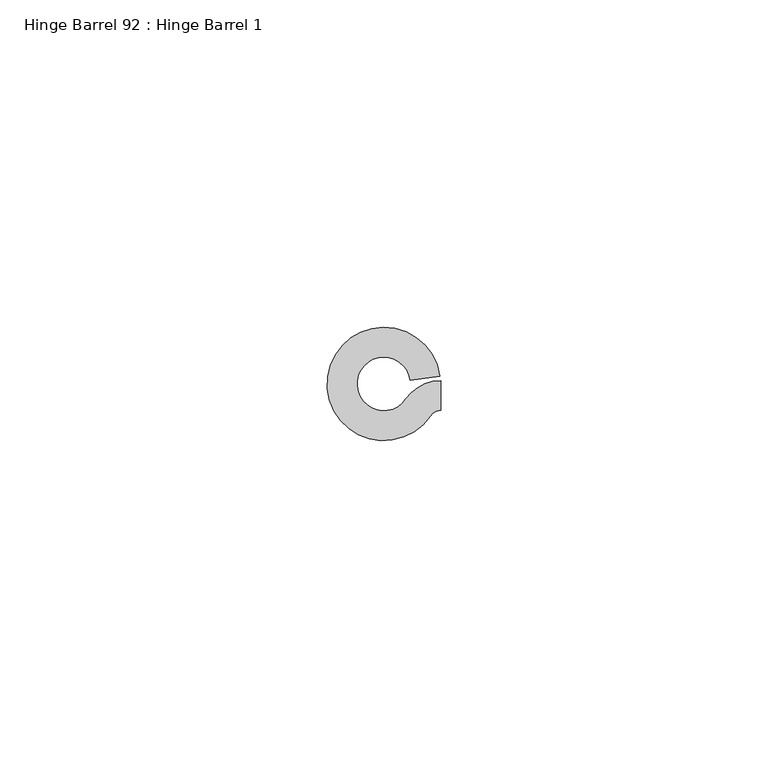
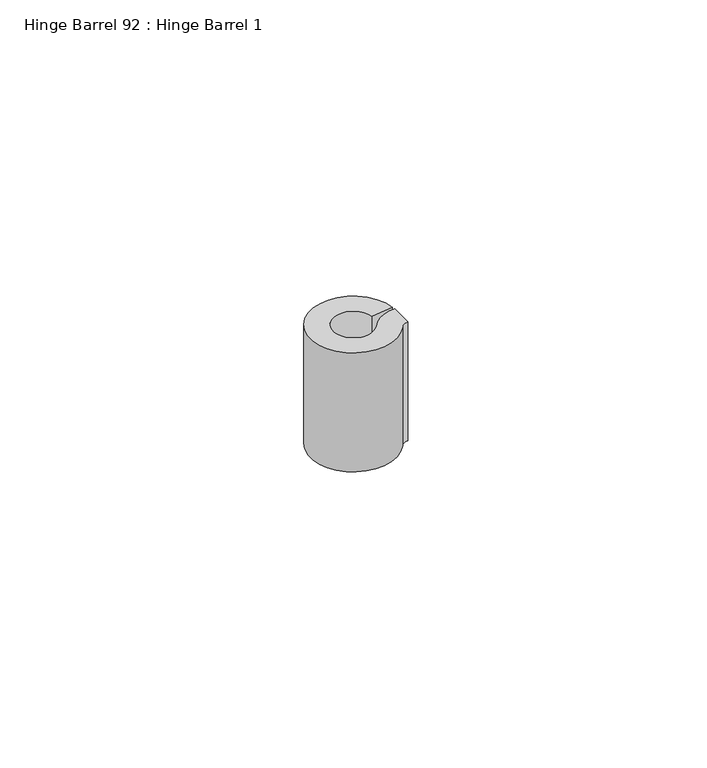
"""IFC4 building model written with IfcOpenShell, lengths in millimetres: proxy geometry, Hinge Barrel 92 : Hinge Barrel 1."""

from ifc_helpers import new_model, si_unit, point, frame, frame_2d, origin, place, context, project, spatial, polyline, circle_curve, trimmed, segment, composite_curve, outline, extrude, source, transform, mapped, element, save


def hinge_barrel_92_hinge_barrel_1_75b3f5ff(model_context):
    return source(origin(), model_context, "Body", "SweptSolid", [
        extrude(outline(composite_curve([segment(trimmed(circle_curve(frame_2d((587327.8245257, -533990.5568067)), 6.4044851), [point((587322.5194669, -533986.9688017))], [point((587327.8245257, -533984.1523216))], False, "CARTESIAN"), True, "CONTINUOUS"), segment(polyline([(587327.8245257, -533984.1523216), (587327.8245257, -533988.7163841)]), True, "CONTINUOUS"), segment(trimmed(circle_curve(frame_2d((587327.8245257, -533990.5568067)), 1.8404226), [point((587327.8245257, -533988.7163841))], [point((587326.3000393, -533989.5257409))], True, "CARTESIAN"), True, "CONTINUOUS"), segment(trimmed(circle_curve(frame_2d((587319.1320739, -533984.6777841)), 8.6534625), [point((587326.3000393, -533989.5257409))], [point((587327.7022899, -533983.4803654))], False, "CARTESIAN"), True, "CONTINUOUS"), segment(polyline([(587327.7022899, -533983.4803654), (587323.1821338, -533984.1119153)]), True, "CONTINUOUS"), segment(trimmed(circle_curve(frame_2d((587319.1320739, -533984.6777841)), 4.0894), [point((587323.1821338, -533984.1119153))], [point((587322.5194669, -533986.9688017))], True, "CARTESIAN"), True, "CONTINUOUS")], self_intersect=False)), frame((0.0, 0.0, 336.55), z_axis=(0.0, 0.0, 1.0), x_axis=(1.0, 0.0, 0.0)), (0.0, 0.0, 1.0), 25.4),
    ])


if __name__ == "__main__":
    model = new_model("IFC4")
    model_context = context("Model", 3, world=origin())
    ifc_project = project(units=[si_unit("LENGTHUNIT", "METRE", prefix="MILLI")], contexts=[model_context])
    site = spatial("IfcSite", under=ifc_project)
    building = spatial("IfcBuilding", under=site)
    placement = place(None, origin())
    hinge_barrel_92_hinge_barrel_1_shape = hinge_barrel_92_hinge_barrel_1_75b3f5ff(model_context)
    element("IfcBuildingElementProxy", 1, Name="Hinge Barrel 92 : Hinge Barrel 1", ObjectType="Hinge Barrel 92 : Hinge Barrel 1", at=placement, inside=building, context=model_context, shape_type="MappedRepresentation", body=[
        mapped(hinge_barrel_92_hinge_barrel_1_shape, transform((0.0, 0.0, 0.0), x_axis=(1.0, 0.0, 0.0), y_axis=(0.0, 1.0, 0.0), z_axis=(0.0, 0.0, 1.0))),
    ])
    save(model, "model.ifc")

# Revit data of these elements
# Element 1 (IfcBuildingElementProxy, "Hinge Barrel 92 : Hinge Barrel 1")
#   Materials on its faces: "6\"X6\" WELD-ON STL BUTT HINGE"
# Materials
#   "6\"X6\" WELD-ON STL BUTT HINGE": class "Metal", colour RGB 189 187 185, transparency 0, Description = "Carbon steel", Cost = 0
